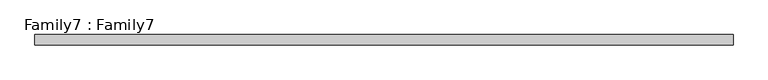
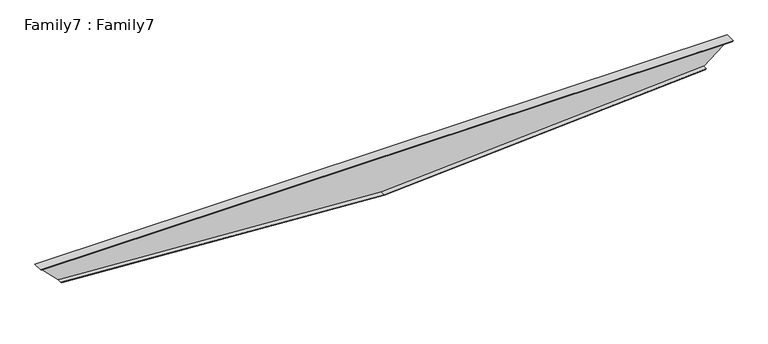
"""IFC4 building model written with IfcOpenShell, lengths in millimetres: beam geometry, Family7 : Family7."""

from ifc_helpers import new_model, si_unit, frame, origin, place, context, project, spatial, polyline, outline, extrude, source, transform, mapped, element, save


def family7_family7_28826eb8(model_context):
    return source(origin(), model_context, "Body", "SweptSolid", [
        extrude(outline(polyline([(-914.4, -14597.6875998), (-1828.8, 0.0), (-914.4, 14561.0062653), (-31.75, 15732.3223771), (-31.75, -15480.3375998), (-914.4, -14597.6875998)])), frame((0.0, -15.875, 0.0), z_axis=(0.0, 1.0, 0.0), x_axis=(0.0, 0.0, 1.0)), (0.0, 0.0, 1.0), 31.75),
        extrude(outline(polyline([(-914.4, 14561.0062653), (-1828.8, 0.0), (-914.4, -14597.6875998), (-948.3381144, -14563.7494854), (-1860.6123856, 0.0025001), (-949.1046767, 14514.9516039), (-914.4, 14561.0062653)])), frame((0.0, -228.6, 0.0), z_axis=(0.0, 1.0, 0.0), x_axis=(0.0, 0.0, 1.0)), (0.0, 0.0, 1.0), 457.2),
        extrude(outline(polyline([(-31.75, 15732.3223771), (0.0, 15774.4560502), (0.0, -15512.0875998), (-31.75, -15480.3375998), (-31.75, 15732.3223771)])), frame((0.0, -228.6, 0.0), z_axis=(0.0, 1.0, 0.0), x_axis=(0.0, 0.0, 1.0)), (0.0, 0.0, 1.0), 457.2),
    ])


if __name__ == "__main__":
    model = new_model("IFC4")
    model_context = context("Model", 3, world=origin())
    ifc_project = project(units=[si_unit("LENGTHUNIT", "METRE", prefix="MILLI")], contexts=[model_context])
    site = spatial("IfcSite", under=ifc_project)
    building = spatial("IfcBuilding", under=site)
    placement = place(None, origin())
    family7_family7_shape = family7_family7_28826eb8(model_context)
    element("IfcBeam", 1, ObjectType="Family7 : Family7", at=placement, inside=building, context=model_context, shape_type="MappedRepresentation", body=[
        mapped(family7_family7_shape, transform((0.0, 0.0, 0.0), x_axis=(1.0, 0.0, 0.0), y_axis=(0.0, 1.0, 0.0), z_axis=(0.0, 0.0, 1.0))),
    ])
    save(model, "model.ifc")

# Revit data of these elements
# Type "Family7 : Family7"
#   Width = 1' - 6"
#   Web_Thickness = 0' - 1 1/4"
#   Length [instance default] = 69' - 10"
#   Depth_Mid [instance default] = 6' - 0"
#   Depth_End = 3' - 0"
#   Angle_Right = 53.00°
#   Angle_Left = 45.00°
#   Structural Material [instance default] = none
# Element 1 (IfcBeam, "Family7 : Family7")
#   Structural Material = Steel
#   Materials on its faces: "Steel"
# Materials
#   "Steel": class "Metal", colour RGB 118 118 114, transparency 0, Description = "Steel, mill finish", Cost = 0
